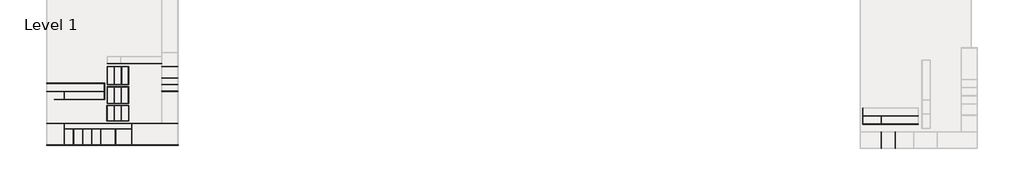
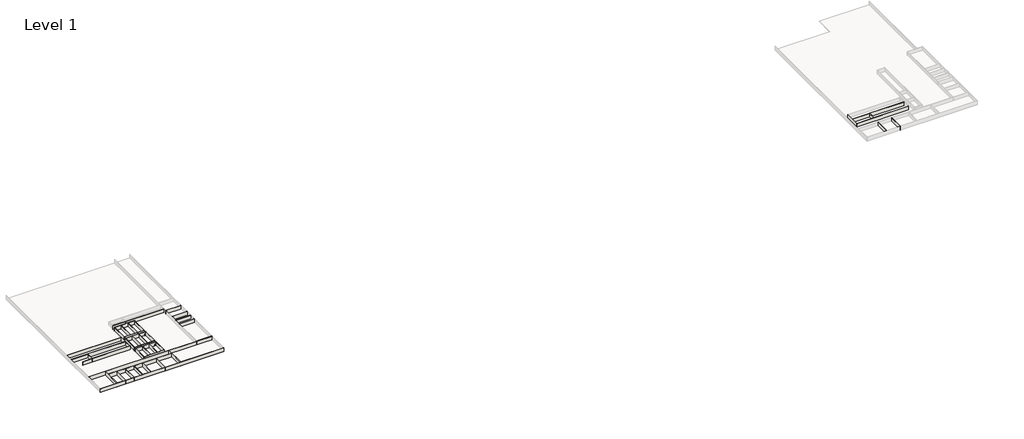
# One storey, part 1 of 4: 45 walls, 12 doors.
"""IFC4 building model written with IfcOpenShell, lengths in millimetres."""

import ifcopenshell
import ifcopenshell.guid

model = None  # the IFC model being written
_history = None  # IfcOwnerHistory: only IFC2X3 demands one
_inside = {}  # id of a spatial element -> (the spatial element, [elements in it])
_under = {}  # id of a project, library or spatial element -> (it, [spatial elements below it])
_declared = {}  # id of a project -> (the project, [libraries it declares])
_typed = {}  # id of a type object -> (the type object, [elements of that type])
_made_of = {}  # id of a material, layer set ... -> (it, [elements and type objects made of it])


def new_model(schema):
    """Start an empty IFC model of exactly this schema.

    Asked for "IFC4X3", IfcOpenShell would pick the latest addendum, in which some entities
    have other attributes; the version numbers below select the first issue.
    IFC2X3 requires an IfcOwnerHistory on every rooted entity: one is made here for all.
    """
    global model, _history
    if schema == "IFC4X3":
        model = ifcopenshell.file(schema_version=(4, 3, 0, 0))
    else:
        model = ifcopenshell.file(schema=schema)
    _inside.clear()
    _under.clear()
    _declared.clear()
    _typed.clear()
    _made_of.clear()
    _history = None
    if model.schema == "IFC2X3":
        org = make("IfcOrganization", Name="unknown")
        user = make(
            "IfcPersonAndOrganization",
            ThePerson=make("IfcPerson", FamilyName="unknown"),
            TheOrganization=org,
        )
        app = make(
            "IfcApplication",
            ApplicationDeveloper=org,
            Version="unknown",
            ApplicationFullName="unknown",
            ApplicationIdentifier="unknown",
        )
        _history = make(
            "IfcOwnerHistory",
            OwningUser=user,
            OwningApplication=app,
            ChangeAction="ADDED",
            CreationDate=0,
        )
    return model


def make(cls, **values):
    """One entity of the class cls with the attributes given. An attribute that is None is left unset."""
    return model.create_entity(
        cls, **{name: value for name, value in values.items() if value is not None}
    )


def rooted(cls, **values):
    """An entity with a GlobalId (a new one), such as an element, a storey or a relation."""
    return make(cls, GlobalId=ifcopenshell.guid.new(), OwnerHistory=_history, **values)


def si_unit(unit_type, name, prefix=None):
    """IfcSIUnit, for example si_unit("LENGTHUNIT", "METRE", prefix="MILLI")."""
    return make("IfcSIUnit", UnitType=unit_type, Prefix=prefix, Name=name)


def assignment(units):
    """IfcUnitAssignment: the units of a project."""
    return None if units is None else make("IfcUnitAssignment", Units=units)


def point(xyz):
    """IfcCartesianPoint."""
    return None if xyz is None else make("IfcCartesianPoint", Coordinates=xyz)


def direction(xyz):
    """IfcDirection."""
    return None if xyz is None else make("IfcDirection", DirectionRatios=xyz)


def frame(location, z_axis=None, x_axis=None):
    """IfcAxis2Placement3D, a coordinate frame: its origin and axes. An axis left out is left unset."""
    return make(
        "IfcAxis2Placement3D",
        Location=point(location),
        Axis=direction(z_axis),
        RefDirection=direction(x_axis),
    )


def origin():
    """The frame at (0, 0, 0) with its axes left unset."""
    return frame((0.0, 0.0, 0.0))


def origin_with_axes():
    """The frame at (0, 0, 0) with the z axis (0, 0, 1) and the x axis (1, 0, 0) written out."""
    return frame((0.0, 0.0, 0.0), z_axis=(0.0, 0.0, 1.0), x_axis=(1.0, 0.0, 0.0))


def place(relative_to, where):
    """IfcLocalPlacement: puts the frame where relative to a parent placement (None: the world)."""
    return make(
        "IfcLocalPlacement", PlacementRelTo=relative_to, RelativePlacement=where
    )


def context(
    kind, dimensions, precision=None, world=None, true_north=None, identifier=None
):
    """IfcGeometricRepresentationContext, for example the 3D "Model" context."""
    return make(
        "IfcGeometricRepresentationContext",
        ContextIdentifier=identifier,
        ContextType=kind,
        CoordinateSpaceDimension=dimensions,
        Precision=precision,
        WorldCoordinateSystem=world,
        TrueNorth=true_north,
    )


def project(units=None, contexts=None):
    """IfcProject with its units and contexts."""
    return rooted(
        "IfcProject",
        Name="project",
        RepresentationContexts=contexts,
        UnitsInContext=assignment(units),
    )


def spatial(cls, under=None, at=None, **own):
    """A site, building, storey or space (cls), placed at a placement, below another one or the project."""
    s = rooted(cls, ObjectPlacement=at, **own)
    if under is not None:
        _under.setdefault(under.id(), (under, []))[1].append(s)
    return s


def polyline(points):
    """IfcPolyline through the points."""
    return make("IfcPolyline", Points=[point(p) for p in points])


def outline(outer, holes=None, kind="AREA"):
    """IfcArbitraryClosedProfileDef: a profile drawn as a closed curve; with holes, ...WithVoids."""
    if holes is None:
        return make("IfcArbitraryClosedProfileDef", ProfileType=kind, OuterCurve=outer)
    return make(
        "IfcArbitraryProfileDefWithVoids",
        ProfileType=kind,
        OuterCurve=outer,
        InnerCurves=holes,
    )


def extrude(swept, where, along, depth):
    """IfcExtrudedAreaSolid: the profile swept, set in the frame where, extruded along a direction by depth."""
    return make(
        "IfcExtrudedAreaSolid",
        SweptArea=swept,
        Position=where,
        ExtrudedDirection=direction(along),
        Depth=depth,
    )


def faces_of(points, faces, orient=None, outer=None):
    """IfcFace entities. A face is a list of loops; a loop is a list of indices into points, from 0.

    orient and outer hold one flag for each loop. By default every Orientation is true, the
    first loop of a face is its IfcFaceOuterBound and the others are IfcFaceBound.
    """
    made = []
    for i, loops in enumerate(faces):
        bounds = []
        for j, loop in enumerate(loops):
            is_outer = j == 0 if outer is None else outer[i][j]
            bounds.append(
                make(
                    "IfcFaceOuterBound" if is_outer else "IfcFaceBound",
                    Bound=make("IfcPolyLoop", Polygon=[points[k] for k in loop]),
                    Orientation=True if orient is None else orient[i][j],
                )
            )
        made.append(make("IfcFace", Bounds=bounds))
    return made


def faceted_brep(points, faces, orient=None, outer=None, voids=None):
    """IfcFacetedBrep: a solid bounded by flat faces; with voids (closed shells), ...WithVoids."""
    shared = [point(p) for p in points]
    hull = make("IfcClosedShell", CfsFaces=faces_of(shared, faces, orient, outer))
    if voids is None:
        return make("IfcFacetedBrep", Outer=hull)
    return make(
        "IfcFacetedBrepWithVoids",
        Outer=hull,
        Voids=[
            make(cls, CfsFaces=faces_of(shared, fs, o, b)) for cls, fs, o, b in voids
        ],
    )


def shape(context_of_items, identifier, shape_type, items):
    """IfcShapeRepresentation: the items that make up one representation, for example the "Body"."""
    return make(
        "IfcShapeRepresentation",
        ContextOfItems=context_of_items,
        RepresentationIdentifier=identifier,
        RepresentationType=shape_type,
        Items=items,
    )


def source(mapping_origin, context_of_items, identifier, shape_type, items):
    """IfcRepresentationMap: a shape defined once, which mapped items show again and again."""
    return make(
        "IfcRepresentationMap",
        MappingOrigin=mapping_origin,
        MappedRepresentation=shape(context_of_items, identifier, shape_type, items),
    )


def transform(
    local_origin,
    x_axis=None,
    y_axis=None,
    z_axis=None,
    scale=None,
    scale2=None,
    scale3=None,
    uniform=True,
):
    """IfcCartesianTransformationOperator3D, or its non-uniform kind. x_axis, y_axis, z_axis: its Axis1, 2, 3."""
    if uniform:
        return make(
            "IfcCartesianTransformationOperator3D",
            Axis1=direction(x_axis),
            Axis2=direction(y_axis),
            LocalOrigin=point(local_origin),
            Scale=scale,
            Axis3=direction(z_axis),
        )
    return make(
        "IfcCartesianTransformationOperator3DnonUniform",
        Axis1=direction(x_axis),
        Axis2=direction(y_axis),
        LocalOrigin=point(local_origin),
        Scale=scale,
        Axis3=direction(z_axis),
        Scale2=scale2,
        Scale3=scale3,
    )


def mapped(mapping_source, mapping_target):
    """IfcMappedItem: shows the shape of a source again, moved by a transform."""
    return make(
        "IfcMappedItem", MappingSource=mapping_source, MappingTarget=mapping_target
    )


def made_of(thing, what):
    """Note that an element or type object is made of a material, layer set ...; save() writes the relation."""
    if what is not None:
        _made_of.setdefault(what.id(), (what, []))[1].append(thing)
    return thing


def element(
    cls,
    number,
    at=None,
    inside=None,
    cuts=None,
    type_object=None,
    material=None,
    context=None,
    identifier="Body",
    shape_type=None,
    held_by="IfcProductDefinitionShape",
    body=None,
    shapes=None,
    **own,
):
    """One element of the class cls, such as IfcWall. Its Tag is "e" and its number.

    at: its placement. inside: the storey or other place that contains it. cuts: it is an
    opening in that element (IfcRelVoidsElement). A single representation is given by context,
    identifier, shape_type and body (its items); several are given by shapes. held_by: the class
    of the entity that holds the representations. save() writes the other relations.
    """
    e = rooted(cls, Tag="e%d" % number, ObjectPlacement=at, **own)
    if body is not None:
        shapes = [shape(context, identifier, shape_type, body)]
    if shapes is not None:
        e.Representation = make(held_by, Representations=shapes)
    if inside is not None:
        _inside.setdefault(inside.id(), (inside, []))[1].append(e)
    if cuts is not None:
        rooted(
            "IfcRelVoidsElement", RelatingBuildingElement=cuts, RelatedOpeningElement=e
        )
    if type_object is not None:
        _typed.setdefault(type_object.id(), (type_object, []))[1].append(e)
    return made_of(e, material)


def aggregate(whole, parts):
    """IfcRelAggregates: a whole, such as a stair, and the parts it consists of."""
    return rooted("IfcRelAggregates", RelatingObject=whole, RelatedObjects=parts)


def save(model, path):
    """Write the relations noted so far, then the file.

    IfcRelAggregates (storeys below a building ...), IfcRelContainedInSpatialStructure (elements
    in a storey), IfcRelDefinesByType, IfcRelAssociatesMaterial and IfcRelDeclares: one each for
    every whole, place, type object, material and project.
    """
    for whole, parts in _under.values():
        aggregate(whole, parts)
    for where, things in _inside.values():
        rooted(
            "IfcRelContainedInSpatialStructure",
            RelatedElements=things,
            RelatingStructure=where,
        )
    for kind, things in _typed.values():
        rooted("IfcRelDefinesByType", RelatedObjects=things, RelatingType=kind)
    for what, things in _made_of.values():
        rooted("IfcRelAssociatesMaterial", RelatedObjects=things, RelatingMaterial=what)
    for by, libraries in _declared.values():
        rooted("IfcRelDeclares", RelatingContext=by, RelatedDefinitions=libraries)
    model.write(path)


def door_686f89d2(model_context):
    return source(origin(), model_context, "Body", "SweptSolid", [
        extrude(outline(polyline([(2209.8, -533.4), (0.0, -533.4), (0.0, -457.2), (2133.6, -457.2), (2133.6, 457.2), (0.0, 457.2), (0.0, 533.4), (2209.8, 533.4), (2209.8, -533.4)])), frame((0.0, -101.6, 0.0), z_axis=(0.0, 1.0, 0.0), x_axis=(0.0, 0.0, 1.0)), (0.0, 0.0, 1.0), 25.4),
        extrude(outline(polyline([(2209.8, 533.4), (2209.8, -533.4), (0.0, -533.4), (0.0, -457.2), (2133.6, -457.2), (2133.6, 457.2), (0.0, 457.2), (0.0, 533.4), (2209.8, 533.4)])), frame((0.0, 76.2, 0.0), z_axis=(0.0, 1.0, 0.0), x_axis=(0.0, 0.0, 1.0)), (0.0, 0.0, 1.0), 25.4),
        extrude(outline(polyline([(457.2, -25.4), (457.2, -76.2), (-457.2, -76.2), (-457.2, -25.4), (457.2, -25.4)])), origin_with_axes(), (0.0, 0.0, 1.0), 2133.6),
    ])


def door_16372e1c(model_context):
    return source(origin(), model_context, "Body", "SweptSolid", [
        extrude(outline(polyline([(2209.8, -533.4), (0.0, -533.4), (0.0, -457.2), (2133.6, -457.2), (2133.6, 457.2), (0.0, 457.2), (0.0, 533.4), (2209.8, 533.4), (2209.8, -533.4)])), frame((0.0, 76.2, 0.0), z_axis=(0.0, 1.0, 0.0), x_axis=(0.0, 0.0, 1.0)), (0.0, 0.0, 1.0), 25.4),
        extrude(outline(polyline([(2209.8, 533.4), (2209.8, -533.4), (0.0, -533.4), (0.0, -457.2), (2133.6, -457.2), (2133.6, 457.2), (0.0, 457.2), (0.0, 533.4), (2209.8, 533.4)])), frame((0.0, -101.6, 0.0), z_axis=(0.0, 1.0, 0.0), x_axis=(0.0, 0.0, 1.0)), (0.0, 0.0, 1.0), 25.4),
        extrude(outline(polyline([(457.2, 25.4), (-457.2, 25.4), (-457.2, 76.2), (457.2, 76.2), (457.2, 25.4)])), origin_with_axes(), (0.0, 0.0, 1.0), 2133.6),
    ])


model = new_model("IFC4")

# Units and contexts
model_context = context("Model", 3, world=origin())
ifc_project = project(units=[si_unit("LENGTHUNIT", "METRE", prefix="MILLI")], contexts=[model_context])

# Site, building, storey
site = spatial("IfcSite", under=ifc_project)
building = spatial("IfcBuilding", under=site)
storey = spatial("IfcBuildingStorey", under=building, Name="Level 1", Elevation=0.0)

# Doors
placement = place(None, origin())
door_shape = door_686f89d2(model_context)
element("IfcDoor", 1, ObjectType="Single-Flush : 36\" x 84\"", at=placement, inside=storey, context=model_context, shape_type="MappedRepresentation", body=[
    mapped(door_shape, transform((-248006.5777071, -25984.7939366, 0.0), x_axis=(-1.0, 0.0, 0.0), y_axis=(0.0, -1.0, 0.0), z_axis=(0.0, 0.0, 1.0))),
])
element("IfcDoor", 2, ObjectType="Single-Flush : 36\" x 84\"", at=placement, inside=storey, context=model_context, shape_type="MappedRepresentation", body=[
    mapped(door_shape, transform((-225577.5777071, -28626.3939366, 0.0), x_axis=(1.0, 0.0, 0.0), y_axis=(0.0, 1.0, 0.0), z_axis=(0.0, 0.0, 1.0))),
])
element("IfcDoor", 3, ObjectType="Single-Flush : 36\" x 84\"", at=placement, inside=storey, context=model_context, shape_type="MappedRepresentation", body=[
    mapped(door_shape, transform((-248006.5777071, -47371.5939366, 0.0), x_axis=(-1.0, 0.0, 0.0), y_axis=(0.0, -1.0, 0.0), z_axis=(0.0, 0.0, 1.0))),
])
element("IfcDoor", 4, ObjectType="Single-Flush : 36\" x 84\"", at=placement, inside=storey, context=model_context, shape_type="MappedRepresentation", body=[
    mapped(door_shape, transform((-225577.5777071, -49911.5939366, 0.0), x_axis=(1.0, 0.0, 0.0), y_axis=(0.0, 1.0, 0.0), z_axis=(0.0, 0.0, 1.0))),
])
element("IfcDoor", 5, ObjectType="Single-Flush : 36\" x 84\"", at=placement, inside=storey, context=model_context, shape_type="MappedRepresentation", body=[
    mapped(door_shape, transform((-240022.2443738, -25984.7939366, 0.0), x_axis=(-1.0, 0.0, 0.0), y_axis=(0.0, -1.0, 0.0), z_axis=(0.0, 0.0, 1.0))),
])
element("IfcDoor", 6, ObjectType="Single-Flush : 36\" x 84\"", at=placement, inside=storey, context=model_context, shape_type="MappedRepresentation", body=[
    mapped(door_shape, transform((-240022.2443738, -47371.5939366, 0.0), x_axis=(-1.0, 0.0, 0.0), y_axis=(0.0, -1.0, 0.0), z_axis=(0.0, 0.0, 1.0))),
])
door_2_shape = door_16372e1c(model_context)
element("IfcDoor", 7, ObjectType="Single-Flush : 36\" x 84\"", at=placement, inside=storey, context=model_context, shape_type="MappedRepresentation", body=[
    mapped(door_2_shape, transform((-225577.5777071, -25984.7939366, 0.0), x_axis=(1.0, 0.0, 0.0), y_axis=(0.0, 1.0, 0.0), z_axis=(0.0, 0.0, 1.0))),
])
element("IfcDoor", 8, ObjectType="Single-Flush : 36\" x 84\"", at=placement, inside=storey, context=model_context, shape_type="MappedRepresentation", body=[
    mapped(door_2_shape, transform((-248006.5777071, -28626.3939366, 0.0), x_axis=(-1.0, 0.0, 0.0), y_axis=(0.0, -1.0, 0.0), z_axis=(0.0, 0.0, 1.0))),
])
element("IfcDoor", 9, ObjectType="Single-Flush : 36\" x 84\"", at=placement, inside=storey, context=model_context, shape_type="MappedRepresentation", body=[
    mapped(door_2_shape, transform((-225577.5777071, -47371.5939366, 0.0), x_axis=(1.0, 0.0, 0.0), y_axis=(0.0, 1.0, 0.0), z_axis=(0.0, 0.0, 1.0))),
])
element("IfcDoor", 10, ObjectType="Single-Flush : 36\" x 84\"", at=placement, inside=storey, context=model_context, shape_type="MappedRepresentation", body=[
    mapped(door_2_shape, transform((-248006.5777071, -49911.5939366, 0.0), x_axis=(-1.0, 0.0, 0.0), y_axis=(0.0, -1.0, 0.0), z_axis=(0.0, 0.0, 1.0))),
])
element("IfcDoor", 11, ObjectType="Single-Flush : 36\" x 84\"", at=placement, inside=storey, context=model_context, shape_type="MappedRepresentation", body=[
    mapped(door_2_shape, transform((-240022.2443738, -28626.3939366, 0.0), x_axis=(-1.0, 0.0, 0.0), y_axis=(0.0, -1.0, 0.0), z_axis=(0.0, 0.0, 1.0))),
])
element("IfcDoor", 12, ObjectType="Single-Flush : 36\" x 84\"", at=placement, inside=storey, context=model_context, shape_type="MappedRepresentation", body=[
    mapped(door_2_shape, transform((-240022.2443738, -49911.5939366, 0.0), x_axis=(-1.0, 0.0, 0.0), y_axis=(0.0, -1.0, 0.0), z_axis=(0.0, 0.0, 1.0))),
])

# Walls
element("IfcWall", 13, ObjectType="Generic - 6\"", at=placement, inside=storey, context=model_context, shape_type="Brep", body=[
    faceted_brep([(662293.8210536, -70787.2690191, 0.0), (662141.4210536, -70787.2690191, 0.0), (620841.0210536, -70787.2690191, 0.0), (620688.6210536, -70787.2690191, 0.0), (600190.8210536, -70787.2690191, 0.0), (600038.4210536, -70787.2690191, 0.0), (600038.4210536, -70787.2690191, 4572.0), (600190.8210536, -70787.2690191, 4572.0), (620688.6210536, -70787.2690191, 4572.0), (620841.0210536, -70787.2690191, 4572.0), (662141.4210536, -70787.2690191, 4572.0), (662293.8210536, -70787.2690191, 4572.0), (662293.8210536, -70939.6690191, 0.0), (662293.8210536, -70939.6690191, 4572.0), (600038.4210536, -70939.6690191, 4572.0), (600038.4210536, -70939.6690191, 0.0)], [[[0, 1, 2, 3, 4, 5, 6, 7, 8, 9, 10, 11]], [[12, 13, 14, 15]], [[5, 4, 3, 2, 1, 0, 12, 15]], [[11, 10, 9, 8, 7, 6, 14, 13]], [[6, 5, 15, 14]], [[0, 11, 13, 12]]]),
])
element("IfcWall", 14, ObjectType="Generic - 6\"", at=placement, inside=storey, context=model_context, shape_type="Brep", body=[
    faceted_brep([(662141.4210536, -61643.2690191, 0.0), (600190.8210536, -61643.2690191, 0.0), (600190.8210536, -61643.2690191, 4572.0), (662141.4210536, -61643.2690191, 4572.0), (662141.4210536, -61795.6690191, 0.0), (662141.4210536, -61795.6690191, 4572.0), (620841.0210536, -61795.6690191, 4572.0), (620688.6210536, -61795.6690191, 4572.0), (600190.8210536, -61795.6690191, 4572.0), (600190.8210536, -61795.6690191, 0.0), (620688.6210536, -61795.6690191, 0.0), (620841.0210536, -61795.6690191, 0.0)], [[[0, 1, 2, 3]], [[4, 5, 6, 7, 8, 9, 10, 11]], [[1, 0, 4, 11, 10, 9]], [[3, 2, 8, 7, 6, 5]], [[2, 1, 9, 8]], [[0, 3, 5, 4]]]),
])
element("IfcWall", 15, ObjectType="Generic - 6\"", at=placement, inside=storey, context=model_context, shape_type="Brep", body=[
    faceted_brep([(600038.4210536, -52651.6690191, 0.0), (600038.4210536, -70787.2690191, 0.0), (600038.4210536, -70787.2690191, 4572.0), (600038.4210536, -52651.6690191, 4572.0), (600190.8210536, -52651.6690191, 0.0), (600190.8210536, -52651.6690191, 4572.0), (600190.8210536, -61643.2690191, 4572.0), (600190.8210536, -61795.6690191, 4572.0), (600190.8210536, -70787.2690191, 4572.0), (600190.8210536, -70787.2690191, 0.0), (600190.8210536, -61795.6690191, 0.0), (600190.8210536, -61643.2690191, 0.0)], [[[0, 1, 2, 3]], [[4, 5, 6, 7, 8, 9, 10, 11]], [[1, 0, 4, 11, 10, 9]], [[3, 2, 8, 7, 6, 5]], [[0, 3, 5, 4]], [[2, 1, 9, 8]]]),
])
element("IfcWall", 16, ObjectType="Generic - 6\"", at=placement, inside=storey, context=model_context, shape_type="SweptSolid", body=[
    extrude(outline(polyline([(620688.6210536, -70787.2690191), (620688.6210536, -61795.6690191), (620841.0210536, -61795.6690191), (620841.0210536, -70787.2690191), (620688.6210536, -70787.2690191)])), origin_with_axes(), (0.0, 0.0, 1.0), 4572.0),
])
element("IfcWall", 17, ObjectType="Generic - 6\"", at=placement, inside=storey, context=model_context, shape_type="SweptSolid", body=[
    extrude(outline(polyline([(620688.6210536, -97824.0338454), (620688.6210536, -79688.4338454), (620841.0210536, -79688.4338454), (620841.0210536, -97824.0338454), (620688.6210536, -97824.0338454)])), origin_with_axes(), (0.0, 0.0, 1.0), 4572.0),
])
element("IfcWall", 18, ObjectType="Generic - 6\"", at=placement, inside=storey, context=model_context, shape_type="SweptSolid", body=[
    extrude(outline(polyline([(636538.2210536, -97824.0338454), (636538.2210536, -79688.4338454), (636690.6210536, -79688.4338454), (636690.6210536, -97824.0338454), (636538.2210536, -97824.0338454)])), origin_with_axes(), (0.0, 0.0, 1.0), 4572.0),
])
element("IfcWall", 19, ObjectType="Generic - 6\"", at=placement, inside=storey, context=model_context, shape_type="SweptSolid", body=[
    extrude(outline(polyline([(-239293.5777071, -76184.6812497), (-239293.5777071, -94320.2812497), (-239445.9777071, -94320.2812497), (-239445.9777071, -76184.6812497), (-239293.5777071, -76184.6812497)])), origin_with_axes(), (0.0, 0.0, 1.0), 4572.0),
])
element("IfcWall", 20, ObjectType="Generic - 6\"", at=placement, inside=storey, context=model_context, shape_type="Brep", body=[
    faceted_brep([(-251740.3777071, -42899.5164234, 0.0), (-251892.7777071, -42899.5164234, 0.0), (-296752.5777071, -42899.5164234, 0.0), (-296904.9777071, -42899.5164234, 0.0), (-308334.9777071, -42899.5164234, 0.0), (-308334.9777071, -42899.5164234, 4572.0), (-296904.9777071, -42899.5164234, 4572.0), (-296752.5777071, -42899.5164234, 4572.0), (-251892.7777071, -42899.5164234, 4572.0), (-251740.3777071, -42899.5164234, 4572.0), (-251740.3777071, -43051.9164234, 0.0), (-251740.3777071, -43051.9164234, 4572.0), (-308334.9777071, -43051.9164234, 4572.0), (-308334.9777071, -43051.9164234, 0.0)], [[[0, 1, 2, 3, 4, 5, 6, 7, 8, 9]], [[10, 11, 12, 13]], [[4, 3, 2, 1, 0, 10, 13]], [[5, 4, 13, 12]], [[9, 8, 7, 6, 5, 12, 11]], [[0, 9, 11, 10]]]),
])
element("IfcWall", 21, ObjectType="Generic - 6\"", at=placement, inside=storey, context=model_context, shape_type="Brep", body=[
    faceted_brep([(-251892.7777071, -33755.5164234, 0.0), (-316738.9777071, -33755.5164234, 0.0), (-316738.9777071, -33755.5164234, 4572.0), (-251892.7777071, -33755.5164234, 4572.0), (-251892.7777071, -33907.9164234, 0.0), (-251892.7777071, -33907.9164234, 4572.0), (-296752.5777071, -33907.9164234, 4572.0), (-296904.9777071, -33907.9164234, 4572.0), (-316738.9777071, -33907.9164234, 4572.0), (-316738.9777071, -33907.9164234, 0.0), (-296904.9777071, -33907.9164234, 0.0), (-296752.5777071, -33907.9164234, 0.0)], [[[0, 1, 2, 3]], [[4, 5, 6, 7, 8, 9, 10, 11]], [[1, 0, 4, 11, 10, 9]], [[3, 2, 8, 7, 6, 5]], [[0, 3, 5, 4]], [[2, 1, 9, 8]]]),
])
element("IfcWall", 22, ObjectType="Generic - 6\"", at=placement, inside=storey, context=model_context, shape_type="Brep", body=[
    faceted_brep([(-251740.3777071, -24611.5164234, 0.0), (-316738.9777071, -24611.5164234, 0.0), (-316738.9777071, -24611.5164234, 4572.0), (-251740.3777071, -24611.5164234, 4572.0), (-251740.3777071, -24763.9164234, 0.0), (-251740.3777071, -24763.9164234, 4572.0), (-251892.7777071, -24763.9164234, 4572.0), (-316738.9777071, -24763.9164234, 4572.0), (-316738.9777071, -24763.9164234, 0.0), (-251892.7777071, -24763.9164234, 0.0)], [[[0, 1, 2, 3]], [[4, 5, 6, 7, 8, 9]], [[1, 0, 4, 9, 8]], [[3, 2, 7, 6, 5]], [[0, 3, 5, 4]], [[2, 1, 8, 7]]]),
])
element("IfcWall", 23, ObjectType="Generic - 6\"", at=placement, inside=storey, context=model_context, shape_type="Brep", body=[
    faceted_brep([(-187477.5777071, -2337.3939366, 0.0), (-187629.9777071, -2337.3939366, 0.0), (-233452.3777071, -2337.3939366, 0.0), (-233604.7777071, -2337.3939366, 0.0), (-248692.3777071, -2337.3939366, 0.0), (-248844.7777071, -2337.3939366, 0.0), (-248844.7777071, -2337.3939366, 4572.0), (-248692.3777071, -2337.3939366, 4572.0), (-233604.7777071, -2337.3939366, 4572.0), (-233452.3777071, -2337.3939366, 4572.0), (-187629.9777071, -2337.3939366, 4572.0), (-187477.5777071, -2337.3939366, 4572.0), (-187477.5777071, -2489.7939366, 0.0), (-187477.5777071, -2489.7939366, 4572.0), (-248844.7777071, -2489.7939366, 4572.0), (-248844.7777071, -2489.7939366, 0.0)], [[[0, 1, 2, 3, 4, 5, 6, 7, 8, 9, 10, 11]], [[12, 13, 14, 15]], [[5, 4, 3, 2, 1, 0, 12, 15]], [[11, 10, 9, 8, 7, 6, 14, 13]], [[6, 5, 15, 14]], [[0, 11, 13, 12]]]),
])
element("IfcWall", 24, ObjectType="Generic - 6\"", at=placement, inside=storey, context=model_context, shape_type="SweptSolid", body=[
    extrude(outline(polyline([(-296904.9777071, -42899.5164234), (-296904.9777071, -33907.9164234), (-296752.5777071, -33907.9164234), (-296752.5777071, -42899.5164234), (-296904.9777071, -42899.5164234)])), origin_with_axes(), (0.0, 0.0, 1.0), 4572.0),
])
element("IfcWall", 25, ObjectType="Generic - 6\"", at=placement, inside=storey, context=model_context, shape_type="Brep", body=[
    faceted_brep([(-169189.5777071, -94320.2812497, 0.0), (-169341.9777071, -94320.2812497, 0.0), (-221005.5777071, -94320.2812497, 0.0), (-221157.9777071, -94320.2812497, 0.0), (-239293.5777071, -94320.2812497, 0.0), (-239445.9777071, -94320.2812497, 0.0), (-255756.9777071, -94320.2812497, 0.0), (-255909.3777071, -94320.2812497, 0.0), (-266005.8777071, -94320.2812497, 0.0), (-266158.2777071, -94320.2812497, 0.0), (-276254.7777071, -94320.2812497, 0.0), (-276407.1777071, -94320.2812497, 0.0), (-286503.6777071, -94320.2812497, 0.0), (-286656.0777071, -94320.2812497, 0.0), (-296752.5777071, -94320.2812497, 0.0), (-296904.9777071, -94320.2812497, 0.0), (-316738.9777071, -94320.2812497, 0.0), (-316891.3777071, -94320.2812497, 0.0), (-316891.3777071, -94320.2812497, 4572.0), (-316738.9777071, -94320.2812497, 4572.0), (-296904.9777071, -94320.2812497, 4572.0), (-296752.5777071, -94320.2812497, 4572.0), (-286656.0777071, -94320.2812497, 4572.0), (-286503.6777071, -94320.2812497, 4572.0), (-276407.1777071, -94320.2812497, 4572.0), (-276254.7777071, -94320.2812497, 4572.0), (-266158.2777071, -94320.2812497, 4572.0), (-266005.8777071, -94320.2812497, 4572.0), (-255909.3777071, -94320.2812497, 4572.0), (-255756.9777071, -94320.2812497, 4572.0), (-239445.9777071, -94320.2812497, 4572.0), (-239293.5777071, -94320.2812497, 4572.0), (-221157.9777071, -94320.2812497, 4572.0), (-221005.5777071, -94320.2812497, 4572.0), (-169341.9777071, -94320.2812497, 4572.0), (-169189.5777071, -94320.2812497, 4572.0), (-169189.5777071, -94472.6812497, 0.0), (-169189.5777071, -94472.6812497, 4572.0), (-316891.3777071, -94472.6812497, 4572.0), (-316891.3777071, -94472.6812497, 0.0)], [[[0, 1, 2, 3, 4, 5, 6, 7, 8, 9, 10, 11, 12, 13, 14, 15, 16, 17, 18, 19, 20, 21, 22, 23, 24, 25, 26, 27, 28, 29, 30, 31, 32, 33, 34, 35]], [[36, 37, 38, 39]], [[17, 16, 15, 14, 13, 12, 11, 10, 9, 8, 7, 6, 5, 4, 3, 2, 1, 0, 36, 39]], [[35, 34, 33, 32, 31, 30, 29, 28, 27, 26, 25, 24, 23, 22, 21, 20, 19, 18, 38, 37]], [[18, 17, 39, 38]], [[0, 35, 37, 36]]]),
])
element("IfcWall", 26, ObjectType="Generic - 6\"", at=placement, inside=storey, context=model_context, shape_type="Brep", body=[
    faceted_brep([(-169341.9777071, -69936.2812497, 0.0), (-187477.5777071, -69936.2812497, 0.0), (-187553.7777071, -69936.2812497, 0.0), (-187553.7777071, -69936.2812497, 4572.0), (-187477.5777071, -69936.2812497, 4572.0), (-169341.9777071, -69936.2812497, 4572.0), (-169341.9777071, -70088.6812497, 0.0), (-169341.9777071, -70088.6812497, 4572.0), (-187553.7777071, -70088.6812497, 4572.0), (-187553.7777071, -70088.6812497, 0.0)], [[[0, 1, 2, 3, 4, 5]], [[6, 7, 8, 9]], [[2, 1, 0, 6, 9]], [[3, 2, 9, 8]], [[5, 4, 3, 8, 7]], [[0, 5, 7, 6]]]),
])
element("IfcWall", 27, ObjectType="Generic - 6\"", at=placement, inside=storey, context=model_context, shape_type="SweptSolid", body=[
    extrude(outline(polyline([(-286656.0777071, -94320.2812497), (-286656.0777071, -76184.6812497), (-286503.6777071, -76184.6812497), (-286503.6777071, -94320.2812497), (-286656.0777071, -94320.2812497)])), origin_with_axes(), (0.0, 0.0, 1.0), 4572.0),
])
element("IfcWall", 28, ObjectType="Generic - 6\"", at=placement, inside=storey, context=model_context, shape_type="Brep", body=[
    faceted_brep([(-296904.9777071, -70088.6812497, 0.0), (-296904.9777071, -94320.2812497, 0.0), (-296904.9777071, -94320.2812497, 4572.0), (-296904.9777071, -70088.6812497, 4572.0), (-296752.5777071, -70088.6812497, 0.0), (-296752.5777071, -70088.6812497, 4572.0), (-296752.5777071, -76032.2812497, 4572.0), (-296752.5777071, -76184.6812497, 4572.0), (-296752.5777071, -94320.2812497, 4572.0), (-296752.5777071, -94320.2812497, 0.0), (-296752.5777071, -76184.6812497, 0.0), (-296752.5777071, -76032.2812497, 0.0)], [[[0, 1, 2, 3]], [[4, 5, 6, 7, 8, 9, 10, 11]], [[1, 0, 4, 11, 10, 9]], [[3, 2, 8, 7, 6, 5]], [[2, 1, 9, 8]], [[0, 3, 5, 4]]]),
])
element("IfcWall", 29, ObjectType="Generic - 6\"", at=placement, inside=storey, context=model_context, shape_type="Brep", body=[
    faceted_brep([(-251892.7777071, -24763.9164234, 0.0), (-251892.7777071, -33755.5164234, 0.0), (-251892.7777071, -33907.9164234, 0.0), (-251892.7777071, -42899.5164234, 0.0), (-251892.7777071, -42899.5164234, 4572.0), (-251892.7777071, -33907.9164234, 4572.0), (-251892.7777071, -33755.5164234, 4572.0), (-251892.7777071, -24763.9164234, 4572.0), (-251740.3777071, -24763.9164234, 0.0), (-251740.3777071, -24763.9164234, 4572.0), (-251740.3777071, -42899.5164234, 4572.0), (-251740.3777071, -42899.5164234, 0.0)], [[[0, 1, 2, 3, 4, 5, 6, 7]], [[8, 9, 10, 11]], [[3, 2, 1, 0, 8, 11]], [[7, 6, 5, 4, 10, 9]], [[4, 3, 11, 10]], [[0, 7, 9, 8]]]),
])
element("IfcWall", 30, ObjectType="Generic - 6\"", at=placement, inside=storey, context=model_context, shape_type="Brep", body=[
    faceted_brep([(-221157.9777071, -70088.6812497, 0.0), (-221157.9777071, -76032.2812497, 0.0), (-221157.9777071, -76184.6812497, 0.0), (-221157.9777071, -94320.2812497, 0.0), (-221157.9777071, -94320.2812497, 4572.0), (-221157.9777071, -76184.6812497, 4572.0), (-221157.9777071, -76032.2812497, 4572.0), (-221157.9777071, -70088.6812497, 4572.0), (-221005.5777071, -70088.6812497, 0.0), (-221005.5777071, -70088.6812497, 4572.0), (-221005.5777071, -94320.2812497, 4572.0), (-221005.5777071, -94320.2812497, 0.0)], [[[0, 1, 2, 3, 4, 5, 6, 7]], [[8, 9, 10, 11]], [[3, 2, 1, 0, 8, 11]], [[7, 6, 5, 4, 10, 9]], [[4, 3, 11, 10]], [[0, 7, 9, 8]]]),
])
element("IfcWall", 31, ObjectType="Generic - 6\"", at=placement, inside=storey, context=model_context, shape_type="Brep", body=[
    faceted_brep([(-221157.9777071, -76032.2812497, 0.0), (-296752.5777071, -76032.2812497, 0.0), (-296752.5777071, -76032.2812497, 4572.0), (-221157.9777071, -76032.2812497, 4572.0), (-221157.9777071, -76184.6812497, 0.0), (-221157.9777071, -76184.6812497, 4572.0), (-239293.5777071, -76184.6812497, 4572.0), (-239445.9777071, -76184.6812497, 4572.0), (-255756.9777071, -76184.6812497, 4572.0), (-255909.3777071, -76184.6812497, 4572.0), (-266005.8777071, -76184.6812497, 4572.0), (-266158.2777071, -76184.6812497, 4572.0), (-276254.7777071, -76184.6812497, 4572.0), (-276407.1777071, -76184.6812497, 4572.0), (-286503.6777071, -76184.6812497, 4572.0), (-286656.0777071, -76184.6812497, 4572.0), (-296752.5777071, -76184.6812497, 4572.0), (-296752.5777071, -76184.6812497, 0.0), (-286656.0777071, -76184.6812497, 0.0), (-286503.6777071, -76184.6812497, 0.0), (-276407.1777071, -76184.6812497, 0.0), (-276254.7777071, -76184.6812497, 0.0), (-266158.2777071, -76184.6812497, 0.0), (-266005.8777071, -76184.6812497, 0.0), (-255909.3777071, -76184.6812497, 0.0), (-255756.9777071, -76184.6812497, 0.0), (-239445.9777071, -76184.6812497, 0.0), (-239293.5777071, -76184.6812497, 0.0)], [[[0, 1, 2, 3]], [[4, 5, 6, 7, 8, 9, 10, 11, 12, 13, 14, 15, 16, 17, 18, 19, 20, 21, 22, 23, 24, 25, 26, 27]], [[1, 0, 4, 27, 26, 25, 24, 23, 22, 21, 20, 19, 18, 17]], [[3, 2, 16, 15, 14, 13, 12, 11, 10, 9, 8, 7, 6, 5]], [[0, 3, 5, 4]], [[2, 1, 17, 16]]]),
])
element("IfcWall", 32, ObjectType="Generic - 6\"", at=placement, inside=storey, context=model_context, shape_type="SweptSolid", body=[
    extrude(outline(polyline([(-169341.9777071, -18882.2812497), (-187477.5777071, -18882.2812497), (-187477.5777071, -18729.8812497), (-169341.9777071, -18729.8812497), (-169341.9777071, -18882.2812497)])), origin_with_axes(), (0.0, 0.0, 1.0), 4572.0),
])
element("IfcWall", 33, ObjectType="Generic - 6\"", at=placement, inside=storey, context=model_context, shape_type="SweptSolid", body=[
    extrude(outline(polyline([(-240708.0443738, -28702.5939366), (-240708.0443738, -47295.3939366), (-240860.4443738, -47295.3939366), (-240860.4443738, -28702.5939366), (-240708.0443738, -28702.5939366)])), origin_with_axes(), (0.0, 0.0, 1.0), 4572.0),
])
element("IfcWall", 34, ObjectType="Generic - 6\"", at=placement, inside=storey, context=model_context, shape_type="Brep", body=[
    faceted_brep([(-248692.3777071, -47295.3939366, 0.0), (-248692.3777071, -28702.5939366, 0.0), (-248692.3777071, -28550.1939366, 0.0), (-248692.3777071, -28550.1939366, 4572.0), (-248692.3777071, -28702.5939366, 4572.0), (-248692.3777071, -47295.3939366, 4572.0), (-248844.7777071, -47295.3939366, 0.0), (-248844.7777071, -47295.3939366, 4572.0), (-248844.7777071, -28550.1939366, 4572.0), (-248844.7777071, -28550.1939366, 0.0)], [[[0, 1, 2, 3, 4, 5]], [[6, 7, 8, 9]], [[2, 1, 0, 6, 9]], [[5, 4, 3, 8, 7]], [[0, 5, 7, 6]], [[3, 2, 9, 8]]]),
])
element("IfcWall", 35, ObjectType="Generic - 6\"", at=placement, inside=storey, context=model_context, shape_type="Brep", body=[
    faceted_brep([(-248844.7777071, -5842.5939366, 0.0), (-248692.3777071, -5842.5939366, 0.0), (-241012.8443738, -5842.5939366, 0.0), (-240860.4443738, -5842.5939366, 0.0), (-232723.7110404, -5842.5939366, 0.0), (-232571.3110404, -5842.5939366, 0.0), (-224891.7777071, -5842.5939366, 0.0), (-224739.3777071, -5842.5939366, 0.0), (-224739.3777071, -5842.5939366, 4572.0), (-224891.7777071, -5842.5939366, 4572.0), (-232571.3110404, -5842.5939366, 4572.0), (-232723.7110404, -5842.5939366, 4572.0), (-240860.4443738, -5842.5939366, 4572.0), (-241012.8443738, -5842.5939366, 4572.0), (-248692.3777071, -5842.5939366, 4572.0), (-248844.7777071, -5842.5939366, 4572.0), (-248844.7777071, -5690.1939366, 0.0), (-248844.7777071, -5690.1939366, 4572.0), (-224739.3777071, -5690.1939366, 4572.0), (-224739.3777071, -5690.1939366, 0.0)], [[[0, 1, 2, 3, 4, 5, 6, 7, 8, 9, 10, 11, 12, 13, 14, 15]], [[16, 17, 18, 19]], [[7, 6, 5, 4, 3, 2, 1, 0, 16, 19]], [[15, 14, 13, 12, 11, 10, 9, 8, 18, 17]], [[0, 15, 17, 16]], [[8, 7, 19, 18]]]),
])
element("IfcWall", 36, ObjectType="Generic - 6\"", at=placement, inside=storey, context=model_context, shape_type="Brep", body=[
    faceted_brep([(-240479.4443738, -25908.5939366, 2133.6), (-240479.4443738, -25908.5939366, 0.0), (-240860.4443738, -25908.5939366, 0.0), (-241012.8443738, -25908.5939366, 0.0), (-247549.3777071, -25908.5939366, 0.0), (-247549.3777071, -25908.5939366, 2133.6), (-248463.7777071, -25908.5939366, 2133.6), (-248463.7777071, -25908.5939366, 0.0), (-248692.3777071, -25908.5939366, 0.0), (-248844.7777071, -25908.5939366, 0.0), (-248844.7777071, -25908.5939366, 4572.0), (-248692.3777071, -25908.5939366, 4572.0), (-241012.8443738, -25908.5939366, 4572.0), (-240860.4443738, -25908.5939366, 4572.0), (-232723.7110404, -25908.5939366, 4572.0), (-232571.3110404, -25908.5939366, 4572.0), (-224891.7777071, -25908.5939366, 4572.0), (-224891.7777071, -25908.5939366, 0.0), (-225120.3777071, -25908.5939366, 0.0), (-225120.3777071, -25908.5939366, 2133.6), (-226034.7777071, -25908.5939366, 2133.6), (-226034.7777071, -25908.5939366, 0.0), (-232571.3110404, -25908.5939366, 0.0), (-232723.7110404, -25908.5939366, 0.0), (-239565.0443738, -25908.5939366, 0.0), (-239565.0443738, -25908.5939366, 2133.6), (-247549.3777071, -26060.9939366, 0.0), (-240479.4443738, -26060.9939366, 0.0), (-240479.4443738, -26060.9939366, 2133.6), (-239565.0443738, -26060.9939366, 2133.6), (-239565.0443738, -26060.9939366, 0.0), (-226034.7777071, -26060.9939366, 0.0), (-226034.7777071, -26060.9939366, 2133.6), (-225120.3777071, -26060.9939366, 2133.6), (-225120.3777071, -26060.9939366, 0.0), (-224891.7777071, -26060.9939366, 0.0), (-224891.7777071, -26060.9939366, 4572.0), (-248844.7777071, -26060.9939366, 4572.0), (-248844.7777071, -26060.9939366, 0.0), (-248463.7777071, -26060.9939366, 0.0), (-248463.7777071, -26060.9939366, 2133.6), (-247549.3777071, -26060.9939366, 2133.6)], [[[0, 1, 2, 3, 4, 5, 6, 7, 8, 9, 10, 11, 12, 13, 14, 15, 16, 17, 18, 19, 20, 21, 22, 23, 24, 25]], [[26, 27, 28, 29, 30, 31, 32, 33, 34, 35, 36, 37, 38, 39, 40, 41]], [[9, 8, 7, 39, 38]], [[35, 34, 18, 17]], [[4, 3, 2, 1, 27, 26]], [[24, 23, 22, 21, 31, 30]], [[16, 15, 14, 13, 12, 11, 10, 37, 36]], [[10, 9, 38, 37]], [[17, 16, 36, 35]], [[40, 39, 7, 6]], [[41, 40, 6, 5]], [[26, 41, 5, 4]], [[19, 18, 34, 33]], [[20, 19, 33, 32]], [[21, 20, 32, 31]], [[28, 27, 1, 0]], [[29, 28, 0, 25]], [[30, 29, 25, 24]]]),
])
element("IfcWall", 37, ObjectType="Generic - 6\"", at=placement, inside=storey, context=model_context, shape_type="Brep", body=[
    faceted_brep([(-240479.4443738, -28550.1939366, 2133.6), (-240479.4443738, -28550.1939366, 0.0), (-247549.3777071, -28550.1939366, 0.0), (-247549.3777071, -28550.1939366, 2133.6), (-248463.7777071, -28550.1939366, 2133.6), (-248463.7777071, -28550.1939366, 0.0), (-248692.3777071, -28550.1939366, 0.0), (-248692.3777071, -28550.1939366, 4572.0), (-224739.3777071, -28550.1939366, 4572.0), (-224739.3777071, -28550.1939366, 0.0), (-225120.3777071, -28550.1939366, 0.0), (-225120.3777071, -28550.1939366, 2133.6), (-226034.7777071, -28550.1939366, 2133.6), (-226034.7777071, -28550.1939366, 0.0), (-239565.0443738, -28550.1939366, 0.0), (-239565.0443738, -28550.1939366, 2133.6), (-247549.3777071, -28702.5939366, 0.0), (-240860.4443738, -28702.5939366, 0.0), (-240708.0443738, -28702.5939366, 0.0), (-240479.4443738, -28702.5939366, 0.0), (-240479.4443738, -28702.5939366, 2133.6), (-239565.0443738, -28702.5939366, 2133.6), (-239565.0443738, -28702.5939366, 0.0), (-232876.1110404, -28702.5939366, 0.0), (-232723.7110404, -28702.5939366, 0.0), (-226034.7777071, -28702.5939366, 0.0), (-226034.7777071, -28702.5939366, 2133.6), (-225120.3777071, -28702.5939366, 2133.6), (-225120.3777071, -28702.5939366, 0.0), (-224891.7777071, -28702.5939366, 0.0), (-224739.3777071, -28702.5939366, 0.0), (-224739.3777071, -28702.5939366, 4572.0), (-224891.7777071, -28702.5939366, 4572.0), (-232723.7110404, -28702.5939366, 4572.0), (-232876.1110404, -28702.5939366, 4572.0), (-240708.0443738, -28702.5939366, 4572.0), (-240860.4443738, -28702.5939366, 4572.0), (-248692.3777071, -28702.5939366, 4572.0), (-248692.3777071, -28702.5939366, 0.0), (-248463.7777071, -28702.5939366, 0.0), (-248463.7777071, -28702.5939366, 2133.6), (-247549.3777071, -28702.5939366, 2133.6)], [[[0, 1, 2, 3, 4, 5, 6, 7, 8, 9, 10, 11, 12, 13, 14, 15]], [[16, 17, 18, 19, 20, 21, 22, 23, 24, 25, 26, 27, 28, 29, 30, 31, 32, 33, 34, 35, 36, 37, 38, 39, 40, 41]], [[6, 5, 39, 38]], [[30, 29, 28, 10, 9]], [[14, 13, 25, 24, 23, 22]], [[2, 1, 19, 18, 17, 16]], [[8, 7, 37, 36, 35, 34, 33, 32, 31]], [[7, 6, 38, 37]], [[9, 8, 31, 30]], [[40, 39, 5, 4]], [[41, 40, 4, 3]], [[16, 41, 3, 2]], [[11, 10, 28, 27]], [[12, 11, 27, 26]], [[13, 12, 26, 25]], [[20, 19, 1, 0]], [[21, 20, 0, 15]], [[22, 21, 15, 14]]]),
])
element("IfcWall", 38, ObjectType="Generic - 6\"", at=placement, inside=storey, context=model_context, shape_type="Brep", body=[
    faceted_brep([(-240479.4443738, -47295.3939366, 2133.6), (-240479.4443738, -47295.3939366, 0.0), (-240708.0443738, -47295.3939366, 0.0), (-240860.4443738, -47295.3939366, 0.0), (-247549.3777071, -47295.3939366, 0.0), (-247549.3777071, -47295.3939366, 2133.6), (-248463.7777071, -47295.3939366, 2133.6), (-248463.7777071, -47295.3939366, 0.0), (-248692.3777071, -47295.3939366, 0.0), (-248844.7777071, -47295.3939366, 0.0), (-248844.7777071, -47295.3939366, 4572.0), (-248692.3777071, -47295.3939366, 4572.0), (-240860.4443738, -47295.3939366, 4572.0), (-240708.0443738, -47295.3939366, 4572.0), (-232876.1110404, -47295.3939366, 4572.0), (-232723.7110404, -47295.3939366, 4572.0), (-224891.7777071, -47295.3939366, 4572.0), (-224739.3777071, -47295.3939366, 4572.0), (-224739.3777071, -47295.3939366, 0.0), (-224891.7777071, -47295.3939366, 0.0), (-225120.3777071, -47295.3939366, 0.0), (-225120.3777071, -47295.3939366, 2133.6), (-226034.7777071, -47295.3939366, 2133.6), (-226034.7777071, -47295.3939366, 0.0), (-232723.7110404, -47295.3939366, 0.0), (-232876.1110404, -47295.3939366, 0.0), (-239565.0443738, -47295.3939366, 0.0), (-239565.0443738, -47295.3939366, 2133.6), (-247549.3777071, -47447.7939366, 0.0), (-240479.4443738, -47447.7939366, 0.0), (-240479.4443738, -47447.7939366, 2133.6), (-239565.0443738, -47447.7939366, 2133.6), (-239565.0443738, -47447.7939366, 0.0), (-226034.7777071, -47447.7939366, 0.0), (-226034.7777071, -47447.7939366, 2133.6), (-225120.3777071, -47447.7939366, 2133.6), (-225120.3777071, -47447.7939366, 0.0), (-224739.3777071, -47447.7939366, 0.0), (-224739.3777071, -47447.7939366, 4572.0), (-248844.7777071, -47447.7939366, 4572.0), (-248844.7777071, -47447.7939366, 0.0), (-248463.7777071, -47447.7939366, 0.0), (-248463.7777071, -47447.7939366, 2133.6), (-247549.3777071, -47447.7939366, 2133.6)], [[[0, 1, 2, 3, 4, 5, 6, 7, 8, 9, 10, 11, 12, 13, 14, 15, 16, 17, 18, 19, 20, 21, 22, 23, 24, 25, 26, 27]], [[28, 29, 30, 31, 32, 33, 34, 35, 36, 37, 38, 39, 40, 41, 42, 43]], [[37, 36, 20, 19, 18]], [[9, 8, 7, 41, 40]], [[4, 3, 2, 1, 29, 28]], [[26, 25, 24, 23, 33, 32]], [[17, 16, 15, 14, 13, 12, 11, 10, 39, 38]], [[10, 9, 40, 39]], [[18, 17, 38, 37]], [[21, 20, 36, 35]], [[22, 21, 35, 34]], [[23, 22, 34, 33]], [[42, 41, 7, 6]], [[43, 42, 6, 5]], [[28, 43, 5, 4]], [[30, 29, 1, 0]], [[31, 30, 0, 27]], [[32, 31, 27, 26]]]),
])
element("IfcWall", 39, ObjectType="Generic - 6\"", at=placement, inside=storey, context=model_context, shape_type="SweptSolid", body=[
    extrude(outline(polyline([(-240860.4443738, -5842.5939366), (-240860.4443738, -25908.5939366), (-241012.8443738, -25908.5939366), (-241012.8443738, -5842.5939366), (-240860.4443738, -5842.5939366)])), origin_with_axes(), (0.0, 0.0, 1.0), 4572.0),
])
element("IfcWall", 40, ObjectType="Generic - 6\"", at=placement, inside=storey, context=model_context, shape_type="SweptSolid", body=[
    extrude(outline(polyline([(-248692.3777071, -5842.5939366), (-248692.3777071, -25908.5939366), (-248844.7777071, -25908.5939366), (-248844.7777071, -5842.5939366), (-248692.3777071, -5842.5939366)])), origin_with_axes(), (0.0, 0.0, 1.0), 4572.0),
])
element("IfcWall", 41, ObjectType="Generic - 6\"", at=placement, inside=storey, context=model_context, shape_type="SweptSolid", body=[
    extrude(outline(polyline([(-276407.1777071, -94320.2812497), (-276407.1777071, -76184.6812497), (-276254.7777071, -76184.6812497), (-276254.7777071, -94320.2812497), (-276407.1777071, -94320.2812497)])), origin_with_axes(), (0.0, 0.0, 1.0), 4572.0),
])
element("IfcWall", 42, ObjectType="Generic - 6\"", at=placement, inside=storey, context=model_context, shape_type="SweptSolid", body=[
    extrude(outline(polyline([(-266158.2777071, -94320.2812497), (-266158.2777071, -76184.6812497), (-266005.8777071, -76184.6812497), (-266005.8777071, -94320.2812497), (-266158.2777071, -94320.2812497)])), origin_with_axes(), (0.0, 0.0, 1.0), 4572.0),
])
element("IfcWall", 43, ObjectType="Generic - 6\"", at=placement, inside=storey, context=model_context, shape_type="SweptSolid", body=[
    extrude(outline(polyline([(-255909.3777071, -94320.2812497), (-255909.3777071, -76184.6812497), (-255756.9777071, -76184.6812497), (-255756.9777071, -94320.2812497), (-255909.3777071, -94320.2812497)])), origin_with_axes(), (0.0, 0.0, 1.0), 4572.0),
])
element("IfcWall", 44, ObjectType="Generic - 6\"", at=placement, inside=storey, context=model_context, shape_type="Brep", body=[
    faceted_brep([(-248844.7777071, -67193.0812497, 0.0), (-248844.7777071, -67040.6812497, 0.0), (-248844.7777071, -49987.7939366, 0.0), (-248844.7777071, -49835.3939366, 0.0), (-248844.7777071, -49835.3939366, 4572.0), (-248844.7777071, -49987.7939366, 4572.0), (-248844.7777071, -67040.6812497, 4572.0), (-248844.7777071, -67193.0812497, 4572.0), (-248997.1777071, -67193.0812497, 0.0), (-248997.1777071, -67193.0812497, 4572.0), (-248997.1777071, -49835.3939366, 4572.0), (-248997.1777071, -49835.3939366, 0.0)], [[[0, 1, 2, 3, 4, 5, 6, 7]], [[8, 9, 10, 11]], [[3, 2, 1, 0, 8, 11]], [[7, 6, 5, 4, 10, 9]], [[4, 3, 11, 10]], [[0, 7, 9, 8]]]),
])
element("IfcWall", 45, ObjectType="Generic - 6\"", at=placement, inside=storey, context=model_context, shape_type="Brep", body=[
    faceted_brep([(-240479.4443738, -49835.3939366, 2133.6), (-240479.4443738, -49835.3939366, 0.0), (-247549.3777071, -49835.3939366, 0.0), (-247549.3777071, -49835.3939366, 2133.6), (-248463.7777071, -49835.3939366, 2133.6), (-248463.7777071, -49835.3939366, 0.0), (-248844.7777071, -49835.3939366, 0.0), (-248844.7777071, -49835.3939366, 4572.0), (-224586.9777071, -49835.3939366, 4572.0), (-224586.9777071, -49835.3939366, 0.0), (-225120.3777071, -49835.3939366, 0.0), (-225120.3777071, -49835.3939366, 2133.6), (-226034.7777071, -49835.3939366, 2133.6), (-226034.7777071, -49835.3939366, 0.0), (-239565.0443738, -49835.3939366, 0.0), (-239565.0443738, -49835.3939366, 2133.6), (-247549.3777071, -49987.7939366, 0.0), (-240860.4443738, -49987.7939366, 0.0), (-240708.0443738, -49987.7939366, 0.0), (-240479.4443738, -49987.7939366, 0.0), (-240479.4443738, -49987.7939366, 2133.6), (-239565.0443738, -49987.7939366, 2133.6), (-239565.0443738, -49987.7939366, 0.0), (-232876.1110404, -49987.7939366, 0.0), (-232723.7110404, -49987.7939366, 0.0), (-226034.7777071, -49987.7939366, 0.0), (-226034.7777071, -49987.7939366, 2133.6), (-225120.3777071, -49987.7939366, 2133.6), (-225120.3777071, -49987.7939366, 0.0), (-224739.3777071, -49987.7939366, 0.0), (-224586.9777071, -49987.7939366, 0.0), (-224586.9777071, -49987.7939366, 4572.0), (-224739.3777071, -49987.7939366, 4572.0), (-232723.7110404, -49987.7939366, 4572.0), (-232876.1110404, -49987.7939366, 4572.0), (-240708.0443738, -49987.7939366, 4572.0), (-240860.4443738, -49987.7939366, 4572.0), (-248844.7777071, -49987.7939366, 4572.0), (-248844.7777071, -49987.7939366, 0.0), (-248463.7777071, -49987.7939366, 0.0), (-248463.7777071, -49987.7939366, 2133.6), (-247549.3777071, -49987.7939366, 2133.6)], [[[0, 1, 2, 3, 4, 5, 6, 7, 8, 9, 10, 11, 12, 13, 14, 15]], [[16, 17, 18, 19, 20, 21, 22, 23, 24, 25, 26, 27, 28, 29, 30, 31, 32, 33, 34, 35, 36, 37, 38, 39, 40, 41]], [[30, 29, 28, 10, 9]], [[6, 5, 39, 38]], [[14, 13, 25, 24, 23, 22]], [[2, 1, 19, 18, 17, 16]], [[8, 7, 37, 36, 35, 34, 33, 32, 31]], [[7, 6, 38, 37]], [[9, 8, 31, 30]], [[11, 10, 28, 27]], [[12, 11, 27, 26]], [[13, 12, 26, 25]], [[40, 39, 5, 4]], [[41, 40, 4, 3]], [[16, 41, 3, 2]], [[20, 19, 1, 0]], [[21, 20, 0, 15]], [[22, 21, 15, 14]]]),
])
element("IfcWall", 46, ObjectType="Generic - 6\"", at=placement, inside=storey, context=model_context, shape_type="SweptSolid", body=[
    extrude(outline(polyline([(-224739.3777071, -67040.6812497), (-224739.3777071, -49987.7939366), (-224586.9777071, -49987.7939366), (-224586.9777071, -67040.6812497), (-224739.3777071, -67040.6812497)])), origin_with_axes(), (0.0, 0.0, 1.0), 4572.0),
])
element("IfcWall", 47, ObjectType="Generic - 6\"", at=placement, inside=storey, context=model_context, shape_type="Brep", body=[
    faceted_brep([(-224586.9777071, -67040.6812497, 0.0), (-224739.3777071, -67040.6812497, 0.0), (-232723.7110404, -67040.6812497, 0.0), (-232876.1110404, -67040.6812497, 0.0), (-240708.0443738, -67040.6812497, 0.0), (-240860.4443738, -67040.6812497, 0.0), (-248844.7777071, -67040.6812497, 0.0), (-248844.7777071, -67040.6812497, 4572.0), (-240860.4443738, -67040.6812497, 4572.0), (-240708.0443738, -67040.6812497, 4572.0), (-232876.1110404, -67040.6812497, 4572.0), (-232723.7110404, -67040.6812497, 4572.0), (-224739.3777071, -67040.6812497, 4572.0), (-224586.9777071, -67040.6812497, 4572.0), (-224586.9777071, -67193.0812497, 0.0), (-224586.9777071, -67193.0812497, 4572.0), (-248844.7777071, -67193.0812497, 4572.0), (-248844.7777071, -67193.0812497, 0.0)], [[[0, 1, 2, 3, 4, 5, 6, 7, 8, 9, 10, 11, 12, 13]], [[14, 15, 16, 17]], [[6, 5, 4, 3, 2, 1, 0, 14, 17]], [[13, 12, 11, 10, 9, 8, 7, 16, 15]], [[7, 6, 17, 16]], [[0, 13, 15, 14]]]),
])
element("IfcWall", 48, ObjectType="Generic - 6\"", at=placement, inside=storey, context=model_context, shape_type="SweptSolid", body=[
    extrude(outline(polyline([(-187477.5777071, -5928.2812497), (-169341.9777071, -5928.2812497), (-169341.9777071, -6080.6812497), (-187477.5777071, -6080.6812497), (-187477.5777071, -5928.2812497)])), origin_with_axes(), (0.0, 0.0, 1.0), 4572.0),
])
element("IfcWall", 49, ObjectType="Generic - 6\"", at=placement, inside=storey, context=model_context, shape_type="Brep", body=[
    faceted_brep([(-224891.7777071, -5842.5939366, 0.0), (-224891.7777071, -25908.5939366, 0.0), (-224891.7777071, -26060.9939366, 0.0), (-224891.7777071, -26060.9939366, 4572.0), (-224891.7777071, -25908.5939366, 4572.0), (-224891.7777071, -5842.5939366, 4572.0), (-224739.3777071, -5842.5939366, 0.0), (-224739.3777071, -5842.5939366, 4572.0), (-224739.3777071, -26060.9939366, 4572.0), (-224739.3777071, -26060.9939366, 0.0)], [[[0, 1, 2, 3, 4, 5]], [[6, 7, 8, 9]], [[2, 1, 0, 6, 9]], [[5, 4, 3, 8, 7]], [[3, 2, 9, 8]], [[0, 5, 7, 6]]]),
])
element("IfcWall", 50, ObjectType="Generic - 6\"", at=placement, inside=storey, context=model_context, shape_type="SweptSolid", body=[
    extrude(outline(polyline([(-224891.7777071, -47295.3939366), (-224891.7777071, -28702.5939366), (-224739.3777071, -28702.5939366), (-224739.3777071, -47295.3939366), (-224891.7777071, -47295.3939366)])), origin_with_axes(), (0.0, 0.0, 1.0), 4572.0),
])
element("IfcWall", 51, ObjectType="Generic - 6\"", at=placement, inside=storey, context=model_context, shape_type="SweptSolid", body=[
    extrude(outline(polyline([(-232723.7110404, -28702.5939366), (-232723.7110404, -47295.3939366), (-232876.1110404, -47295.3939366), (-232876.1110404, -28702.5939366), (-232723.7110404, -28702.5939366)])), origin_with_axes(), (0.0, 0.0, 1.0), 4572.0),
])
element("IfcWall", 52, ObjectType="Generic - 6\"", at=placement, inside=storey, context=model_context, shape_type="SweptSolid", body=[
    extrude(outline(polyline([(-232571.3110404, -5842.5939366), (-232571.3110404, -25908.5939366), (-232723.7110404, -25908.5939366), (-232723.7110404, -5842.5939366), (-232571.3110404, -5842.5939366)])), origin_with_axes(), (0.0, 0.0, 1.0), 4572.0),
])
element("IfcWall", 53, ObjectType="Generic - 6\"", at=placement, inside=storey, context=model_context, shape_type="SweptSolid", body=[
    extrude(outline(polyline([(-240708.0443738, -49987.7939366), (-240708.0443738, -67040.6812497), (-240860.4443738, -67040.6812497), (-240860.4443738, -49987.7939366), (-240708.0443738, -49987.7939366)])), origin_with_axes(), (0.0, 0.0, 1.0), 4572.0),
])
element("IfcWall", 54, ObjectType="Generic - 6\"", at=placement, inside=storey, context=model_context, shape_type="SweptSolid", body=[
    extrude(outline(polyline([(-232723.7110404, -49987.7939366), (-232723.7110404, -67040.6812497), (-232876.1110404, -67040.6812497), (-232876.1110404, -49987.7939366), (-232723.7110404, -49987.7939366)])), origin_with_axes(), (0.0, 0.0, 1.0), 4572.0),
])
element("IfcWall", 55, ObjectType="Generic - 6\"", at=placement, inside=storey, context=model_context, shape_type="SweptSolid", body=[
    extrude(outline(polyline([(-169341.9777071, -33755.5164234), (-187477.5777071, -33755.5164234), (-187477.5777071, -33603.1164234), (-169341.9777071, -33603.1164234), (-169341.9777071, -33755.5164234)])), origin_with_axes(), (0.0, 0.0, 1.0), 4572.0),
])
element("IfcWall", 56, ObjectType="Generic - 6\"", at=placement, inside=storey, context=model_context, shape_type="SweptSolid", body=[
    extrude(outline(polyline([(-169341.9777071, -26349.8812497), (-187477.5777071, -26349.8812497), (-187477.5777071, -26197.4812497), (-169341.9777071, -26197.4812497), (-169341.9777071, -26349.8812497)])), origin_with_axes(), (0.0, 0.0, 1.0), 4572.0),
])
element("IfcWall", 57, ObjectType="Generic - 6\"", at=placement, inside=storey, context=model_context, shape_type="Brep", body=[
    faceted_brep([(-187553.7777071, -69936.2812497, 0.0), (-187629.9777071, -69936.2812497, 0.0), (-316738.9777071, -69936.2812497, 0.0), (-316738.9777071, -69936.2812497, 4572.0), (-187629.9777071, -69936.2812497, 4572.0), (-187553.7777071, -69936.2812497, 4572.0), (-187553.7777071, -70088.6812497, 0.0), (-187553.7777071, -70088.6812497, 4572.0), (-221005.5777071, -70088.6812497, 4572.0), (-221157.9777071, -70088.6812497, 4572.0), (-296752.5777071, -70088.6812497, 4572.0), (-296904.9777071, -70088.6812497, 4572.0), (-316738.9777071, -70088.6812497, 4572.0), (-316738.9777071, -70088.6812497, 0.0), (-296904.9777071, -70088.6812497, 0.0), (-296752.5777071, -70088.6812497, 0.0), (-221157.9777071, -70088.6812497, 0.0), (-221005.5777071, -70088.6812497, 0.0)], [[[0, 1, 2, 3, 4, 5]], [[6, 7, 8, 9, 10, 11, 12, 13, 14, 15, 16, 17]], [[2, 1, 0, 6, 17, 16, 15, 14, 13]], [[5, 4, 3, 12, 11, 10, 9, 8, 7]], [[0, 5, 7, 6]], [[3, 2, 13, 12]]]),
])

save(model, "model.ifc")

# Revit data of these elements
# Project information
#   Project Issue Date = "Issue Date"
#   Project Status = "Project Status"
#   Client Name = "Owner"
#   Project Address = "Enter address here"
#   Project Name = "Xcel Sports Complex - Jackson"
#   Project Number = "Project Number"
# Type "Single-Flush : 36\" x 84\""
#   Type Mark = "1"
#   Assembly Code = "C1020"
#   Thickness = 0.166667 ft
#   Height = 7.00 ft
#   Trim Projection Ext = 0.083333 ft
#   Trim Projection Int = 0.083333 ft
#   Trim Width = 0.25 ft
#   Width = 3.00 ft
#   Door Material = Door - Panel
#   Frame Material = Door - Frame
#   Function = (empty or 0)
#   Wall Closure = (empty or 0)
# Type "Generic - 6\""
#   Assembly Code = "B2010"
#   Width = 0.50 ft
#   Layers, outside or top first: 0.50 ft no material (function 1)
# Elements 1, 2, 3, 4, 5, 6, 7, 8, 9, 10, 11, 12 (IfcDoor, "Single-Flush : 36\" x 84\"")
#   Phase Created = New Construction
#   Materials on its faces: "Door - Frame", "Door - Panel"
# Elements 13, 14, 15, 16, 17, 18, 19, 20, 21, 22, 23, 24, 25, 26, 27, 28, 29, 30, 31, 32, 33, 34, 35, 36, 37, 38, 39, 40, 41, 42, 43, 44, 45, 46, 47, 48, 49, 50, 51, 52, 53, 54, 55, 56, 57 (IfcWall, "Generic - 6\"")
#   Top Offset = 0.00 ft
#   Base Offset = 0.00 ft
#   wall height = 15.00 ft
#   Phase Created = New Construction
#   Base Constraint = Level 1
#   Top Constraint = Level 2
#   Materials on its faces: "Default Wall"
# Materials
#   "Door - Panel": class "Wood", colour RGB 114 82 51, transparency 0
#   "Door - Frame": class "Miscellaneous", colour RGB 153 76 43, transparency 0
#   "Default Wall": class "Miscellaneous", colour RGB 80 80 80, transparency 0
# Room, not placed, phase "New Construction", upper offset 0.00 ft, lower offset 0.00 ft
#   Number = "191"
#   Name = "LOCKER ROOM"
# Room, not placed, phase "New Construction", upper offset 0.00 ft, lower offset 0.00 ft
#   Number = "192"
#   Name = "LOCKER ROOM"
# Room at (2501431.959, -5033.857) mm, phase "New Construction", upper level "Level 1", upper offset 10.00 ft, lower offset 0.00 ft
#   Number = "151"
#   Name = "FLEX SPACE"
# Room at (2507554.629, 25361.374) mm, phase "New Construction", upper level "Level 1", upper offset 10.00 ft, lower offset 0.00 ft
#   Number = "152"
#   Name = "FLEX SPACE"
# Room at (2501431.959, 55446.338) mm, phase "New Construction", upper level "Level 1", upper offset 10.00 ft, lower offset 0.00 ft
#   Number = "153"
#   Name = "FLEX SPACE"
# Room at (2504769.519, 85014.455) mm, phase "New Construction", upper level "Level 1", upper offset 10.00 ft, lower offset 0.00 ft
#   Number = "154"
#   Name = "FLEX SPACE"
# Room at (2501416.719, 5700.078) mm, phase "New Construction", upper level "Level 1", upper offset 10.00 ft, lower offset 0.00 ft
#   Number = "155"
#   Name = "FLEX SPACE"
# Room at (2507830.489, 15889.516) mm, phase "New Construction", upper level "Level 1", upper offset 10.00 ft, lower offset 0.00 ft
#   Number = "156"
#   Name = "FLEX SPACE"
# Room at (2501431.959, 47487.065) mm, phase "New Construction", upper level "Level 1", upper offset 10.00 ft, lower offset 0.00 ft
#   Number = "157"
#   Name = "FLEX SPACE"
# Room at (2504462.954, 93467.114) mm, phase "New Construction", upper level "Level 1", upper offset 10.00 ft, lower offset 0.00 ft
#   Number = "158"
#   Name = "FLEX SPACE"
# Room at (1650111.232, -40892.497) mm, phase "New Construction", upper level "Level 1", upper offset 10.00 ft, lower offset 0.00 ft
#   Number = "51"
#   Name = "CLINIC"
# Room at (1656181.227, -6826.439) mm, phase "New Construction", upper level "Level 1", upper offset 10.00 ft, lower offset 0.00 ft
#   Number = "52"
#   Name = "KITCHEN / CONCESSIONS / OTHER XCEL RETAIL"
# Room at (1656181.227, 34527.786) mm, phase "New Construction", upper level "Level 1", upper offset 10.00 ft, lower offset 0.00 ft
#   Number = "53"
#   Name = "LOCKEROOM"
# Room at (1649995.832, 46297.273) mm, phase "New Construction", upper level "Level 1", upper offset 10.00 ft, lower offset 0.00 ft
#   Number = "54"
#   Name = "CLASSROOM"
# Room at (1649995.832, 16675.676) mm, phase "New Construction", upper level "Level 1", upper offset 10.00 ft, lower offset 0.00 ft
#   Number = "55"
#   Name = "LOBBY/RECEPTION"
# Room at (1540760.606, -52030.077) mm, phase "New Construction", upper level "Level 1", upper offset 10.00 ft, lower offset 0.00 ft
#   Number = "56"
#   Name = "Room"
# Room at (1528845.252, -48632.382) mm, phase "New Construction", upper level "Level 1", upper offset 10.00 ft, lower offset 0.00 ft
#   Number = "57"
#   Name = "STORAGE"
# Room at (1528952.324, 111947.24) mm, phase "New Construction", upper level "Level 1", upper offset 10.00 ft, lower offset 0.00 ft
#   Number = "58"
#   Name = "STORAGE"
# Room at (1537894.321, 116775.918) mm, phase "New Construction", upper level "Level 1", upper offset 10.00 ft, lower offset 0.00 ft
#   Number = "59"
#   Name = "Room"
# Room at (1644602.734, 31454.01) mm, phase "New Construction", upper level "Level 1", upper offset 10.00 ft, lower offset 0.00 ft
#   Number = "60"
#   Name = "LOCKEROOM"
# Room at (1599923.364, -52030.077) mm, phase "New Construction", upper level "Level 1", upper offset 10.00 ft, lower offset 0.00 ft
#   Number = "61"
#   Name = "Room"
# Room at (1607807.943, -48632.382) mm, phase "New Construction", upper level "Level 1", upper offset 10.00 ft, lower offset 0.00 ft
#   Number = "62"
#   Name = "STORAGE"
# Room at (1606634.071, 111947.24) mm, phase "New Construction", upper level "Level 1", upper offset 10.00 ft, lower offset 0.00 ft
#   Number = "63"
